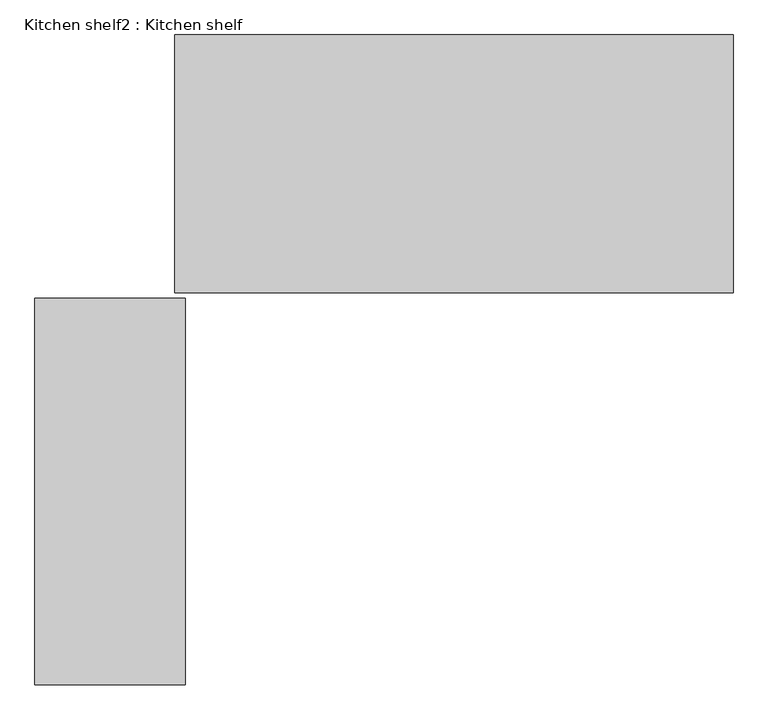
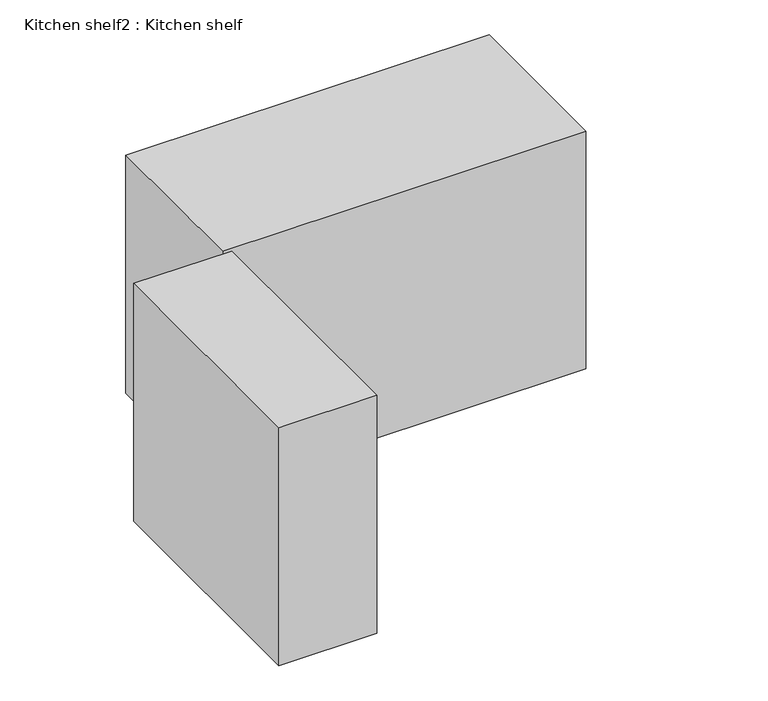
"""IFC4 building model written with IfcOpenShell, lengths in millimetres: furniture geometry, Kitchen shelf2 : Kitchen shelf."""

from ifc_helpers import new_model, si_unit, origin, origin_with_axes, place, context, project, spatial, polyline, outline, extrude, source, transform, mapped, element, save


def kitchen_shelf2_kitchen_shelf_9b1d00cd(model_context):
    return source(origin(), model_context, "Body", "SweptSolid", [
        extrude(outline(polyline([(23025.8870052, 10580.3615366), (23025.8870052, 9665.9615366), (22670.2870052, 9665.9615366), (22670.2870052, 10580.3615366), (23025.8870052, 10580.3615366)])), origin_with_axes(), (0.0, 0.0, 1.0), 914.4),
        extrude(outline(polyline([(24321.2870052, 11202.6615366), (24321.2870052, 10593.0615366), (23000.4870052, 10593.0615366), (23000.4870052, 11202.6615366), (24321.2870052, 11202.6615366)])), origin_with_axes(), (0.0, 0.0, 1.0), 914.4),
    ])


if __name__ == "__main__":
    model = new_model("IFC4")
    model_context = context("Model", 3, world=origin())
    ifc_project = project(units=[si_unit("LENGTHUNIT", "METRE", prefix="MILLI")], contexts=[model_context])
    site = spatial("IfcSite", under=ifc_project)
    building = spatial("IfcBuilding", under=site)
    placement = place(None, origin())
    kitchen_shelf2_kitchen_shelf_shape = kitchen_shelf2_kitchen_shelf_9b1d00cd(model_context)
    element("IfcFurniture", 1, ObjectType="Kitchen shelf2 : Kitchen shelf", at=placement, inside=building, context=model_context, shape_type="MappedRepresentation", body=[
        mapped(kitchen_shelf2_kitchen_shelf_shape, transform((0.0, 0.0, 0.0), x_axis=(1.0, 0.0, 0.0), y_axis=(0.0, 1.0, 0.0), z_axis=(0.0, 0.0, 1.0))),
    ])
    save(model, "model.ifc")

# Revit data of these elements
# Element 1 (IfcFurniture, "Kitchen shelf2 : Kitchen shelf")
#   Materials on its faces: "food"
# Materials
#   "food": class "Glass", colour RGB 233 233 233, transparency 0, Description = "Soda Lime Glass", Cost = 0
